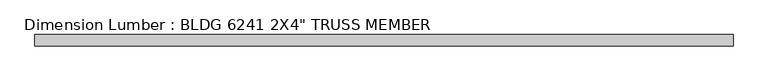
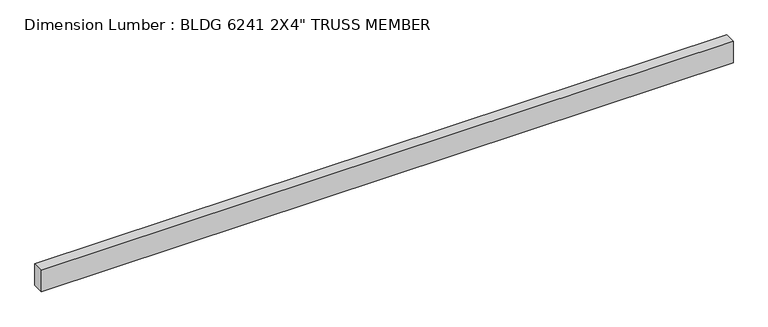
"""IFC4 building model written with IfcOpenShell, lengths in millimetres: beam geometry."""

from ifc_helpers import new_model, si_unit, frame, origin, place, context, project, spatial, polyline, outline, extrude, source, transform, mapped, element, save


def beam_fc8bf4ae(model_context):
    return source(origin(), model_context, "Body", "SweptSolid", [
        extrude(outline(polyline([(1562.6646551, 25.4), (1562.6646551, -25.4), (-1550.1468127, -25.4), (-1550.1468127, 25.4), (1562.6646551, 25.4)])), frame((0.0, 0.0, -50.8), z_axis=(0.0, 0.0, 1.0), x_axis=(1.0, 0.0, 0.0)), (0.0, 0.0, 1.0), 101.6),
    ])


if __name__ == "__main__":
    model = new_model("IFC4")
    model_context = context("Model", 3, world=origin())
    ifc_project = project(units=[si_unit("LENGTHUNIT", "METRE", prefix="MILLI")], contexts=[model_context])
    site = spatial("IfcSite", under=ifc_project)
    building = spatial("IfcBuilding", under=site)
    placement = place(None, origin())
    beam_shape = beam_fc8bf4ae(model_context)
    element("IfcBeam", 1, ObjectType="Dimension Lumber : BLDG 6241 2X4\" TRUSS MEMBER", at=placement, inside=building, context=model_context, shape_type="MappedRepresentation", body=[
        mapped(beam_shape, transform((0.0, 0.0, 0.0), x_axis=(1.0, 0.0, 0.0), y_axis=(0.0, 1.0, 0.0), z_axis=(0.0, 0.0, 1.0))),
    ])
    save(model, "model.ifc")

# Revit data of these elements
# Type "Dimension Lumber : BLDG 6241 2X4\" TRUSS MEMBER"
#   Assembly Code = "B10"
#   A = 0.273472 SF
#   Length [instance default] = 5' - 0"
#   b = 0' - 2"
#   d = 0' - 4"
#   Structural Material [instance default] = Softwood, Lumber
# Element 1 (IfcBeam, "Dimension Lumber : BLDG 6241 2X4\" TRUSS MEMBER")
#   Materials on its faces: "Softwood, Lumber"
# Materials
#   "Softwood, Lumber": class "Wood", colour RGB 223 192 134, transparency 0, Description = "Pinus Echinata", Cost = 0
